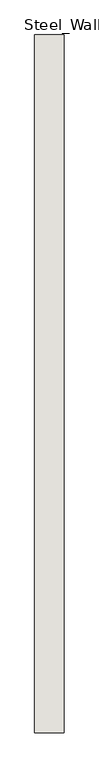
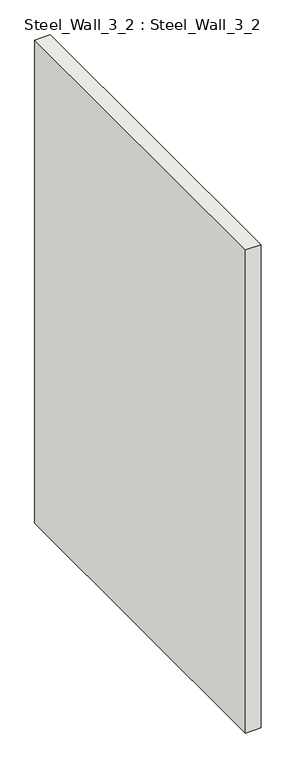
"""IFC4 building model written with IfcOpenShell, lengths in millimetres: wall geometry, Steel_Wall_3_2 : Steel_Wall_3_2."""

from ifc_helpers import new_model, si_unit, frame, origin, place, context, project, spatial, polyline, outline, extrude, source, transform, mapped, element, save


def steel_wall_3_2_steel_wall_3_2_60cdce26(model_context):
    return source(origin(), model_context, "Body", "SweptSolid", [
        extrude(outline(polyline([(215.0, 11955.0), (215.0, 9595.0), (115.0, 9595.0), (115.0, 11955.0), (215.0, 11955.0)])), frame((0.0, 0.0, 250.0), z_axis=(0.0, 0.0, 1.0), x_axis=(1.0, 0.0, 0.0)), (0.0, 0.0, 1.0), 3300.0),
    ])


if __name__ == "__main__":
    model = new_model("IFC4")
    model_context = context("Model", 3, world=origin())
    ifc_project = project(units=[si_unit("LENGTHUNIT", "METRE", prefix="MILLI")], contexts=[model_context])
    site = spatial("IfcSite", under=ifc_project)
    building = spatial("IfcBuilding", under=site)
    placement = place(None, origin())
    steel_wall_3_2_steel_wall_3_2_shape = steel_wall_3_2_steel_wall_3_2_60cdce26(model_context)
    element("IfcWall", 1, ObjectType="Steel_Wall_3_2 : Steel_Wall_3_2", at=placement, inside=building, context=model_context, shape_type="MappedRepresentation", body=[
        mapped(steel_wall_3_2_steel_wall_3_2_shape, transform((0.0, 0.0, 0.0), x_axis=(1.0, 0.0, 0.0), y_axis=(0.0, 1.0, 0.0), z_axis=(0.0, 0.0, 1.0))),
    ])
    save(model, "model.ifc")

# Revit data of these elements
# Type "Steel_Wall_3_2 : Steel_Wall_3_2"
#   NameOverride = "Steel_Wall_3_2"
# Element 1 (IfcWall, "Steel_Wall_3_2 : Steel_Wall_3_2")
#   Materials on its faces: "IfcSurfaceStyle #33"
# Materials
#   "IfcSurfaceStyle #33": class "Unassigned", colour RGB 214 214 214, transparency 0
